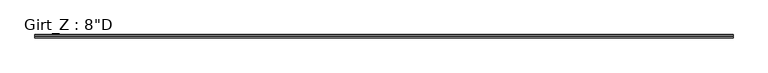
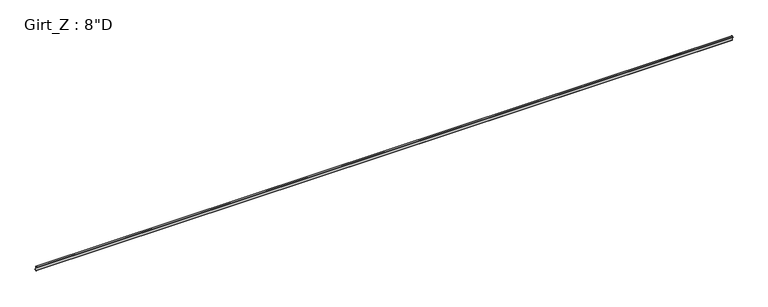
"""IFC4 building model written with IfcOpenShell, lengths in millimetres: beam geometry."""

from ifc_helpers import new_model, si_unit, point, frame, frame_2d, origin, place, context, project, spatial, polyline, circle_curve, trimmed, segment, composite_curve, outline, extrude, source, transform, mapped, element, save


def beam_b3fea3cc(model_context):
    return source(origin(), model_context, "Body", "SweptSolid", [
        extrude(outline(composite_curve([segment(polyline([(-63.5, 101.6), (-3.3734375, 101.6)]), True, "CONTINUOUS"), segment(trimmed(circle_curve(frame_2d((-3.3734375, 96.8375)), 4.7625), [point((-3.3734375, 101.6))], [point((1.3890625, 96.8375))], False, "CARTESIAN"), True, "CONTINUOUS"), segment(polyline([(1.3890625, 96.8375), (1.3890625, -96.8389339)]), True, "CONTINUOUS"), segment(trimmed(circle_curve(frame_2d((3.3748024, -96.8389339)), 1.9857399), [point((1.3890625, -96.8389339))], [point((3.2694106, -98.821875))], True, "CARTESIAN"), True, "CONTINUOUS"), segment(polyline([(3.2694106, -98.821875), (62.204539, -98.821875), (73.6169367, -85.221109), (75.745104, -87.0068534), (63.5, -101.6), (3.3734375, -101.6)]), True, "CONTINUOUS"), segment(trimmed(circle_curve(frame_2d((3.3734375, -96.8375)), 4.7625), [point((3.3734375, -101.6))], [point((-1.3890625, -96.8375))], False, "CARTESIAN"), True, "CONTINUOUS"), segment(polyline([(-1.3890625, -96.8375), (-1.3890625, 96.8381931)]), True, "CONTINUOUS"), segment(trimmed(circle_curve(frame_2d((-3.3741066, 96.8381931)), 1.9850441), [point((-1.3890625, 96.8381931))], [point((-3.3005807, 98.821875))], True, "CARTESIAN"), True, "CONTINUOUS"), segment(polyline([(-3.3005807, 98.821875), (-62.204539, 98.821875), (-73.6169367, 85.221109), (-75.745104, 87.0068534), (-63.5, 101.6)]), True, "CONTINUOUS")], self_intersect=False)), frame((-15595.6, 0.0, 0.0), z_axis=(1.0, 0.0, 0.0), x_axis=(0.0, 1.0, 0.0)), (0.0, 0.0, 1.0), 31191.2),
    ])


if __name__ == "__main__":
    model = new_model("IFC4")
    model_context = context("Model", 3, world=origin())
    ifc_project = project(units=[si_unit("LENGTHUNIT", "METRE", prefix="MILLI")], contexts=[model_context])
    site = spatial("IfcSite", under=ifc_project)
    building = spatial("IfcBuilding", under=site)
    placement = place(None, origin())
    beam_shape = beam_b3fea3cc(model_context)
    element("IfcBeam", 1, ObjectType="Girt_Z : 8\"D", at=placement, inside=building, context=model_context, shape_type="MappedRepresentation", body=[
        mapped(beam_shape, transform((0.0, 0.0, 0.0), x_axis=(1.0, 0.0, 0.0), y_axis=(0.0, 1.0, 0.0), z_axis=(0.0, 0.0, 1.0))),
    ])
    save(model, "model.ifc")

# Revit data of these elements
# Type "Girt_Z : 8\"D"
#   Web_Thickness = 0' - 0 7/64"
#   Length [instance default] = 10' - 0"
#   Leg_1 = 0' - 2 1/2"
#   Height = 0' - 8"
#   Structural Material [instance default] = none
# Element 1 (IfcBeam, "Girt_Z : 8\"D")
#   Structural Material = Steel
#   Materials on its faces: "Steel"
# Materials
#   "Steel": class "Metal", colour RGB 118 118 114, transparency 0, Description = "Steel, mill finish", Cost = 0
